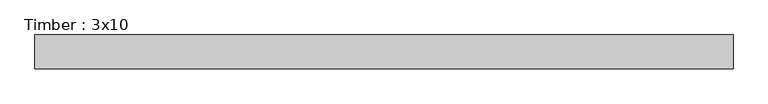
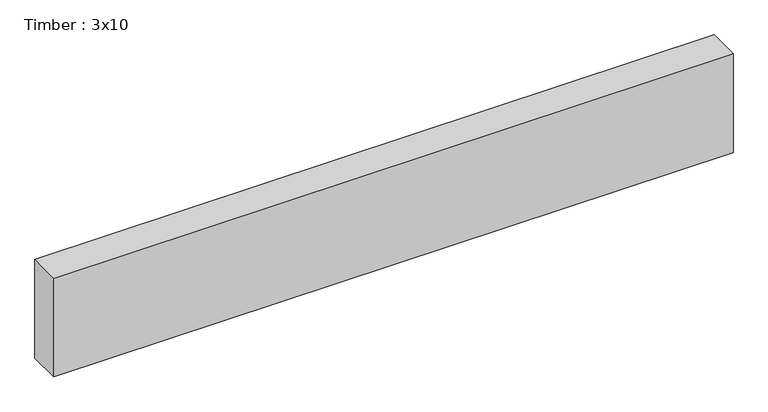
"""IFC4 building model written with IfcOpenShell, lengths in millimetres: beam geometry, Timber : 3x10."""

from ifc_helpers import new_model, si_unit, frame, origin, place, context, project, spatial, polyline, outline, extrude, source, transform, mapped, element, save


def timber_3x10_88a0bdfd(model_context):
    return source(origin(), model_context, "Body", "SweptSolid", [
        extrude(outline(polyline([(785.1325751, 38.1), (785.1325751, -38.1), (-785.1325751, -38.1), (-785.1325751, 38.1), (785.1325751, 38.1)])), frame((0.0, 0.0, -120.65), z_axis=(0.0, 0.0, 1.0), x_axis=(1.0, 0.0, 0.0)), (0.0, 0.0, 1.0), 241.3),
    ])


if __name__ == "__main__":
    model = new_model("IFC4")
    model_context = context("Model", 3, world=origin())
    ifc_project = project(units=[si_unit("LENGTHUNIT", "METRE", prefix="MILLI")], contexts=[model_context])
    site = spatial("IfcSite", under=ifc_project)
    building = spatial("IfcBuilding", under=site)
    placement = place(None, origin())
    timber_3x10_shape = timber_3x10_88a0bdfd(model_context)
    element("IfcBeam", 1, ObjectType="Timber : 3x10", at=placement, inside=building, context=model_context, shape_type="MappedRepresentation", body=[
        mapped(timber_3x10_shape, transform((0.0, 0.0, 0.0), x_axis=(1.0, 0.0, 0.0), y_axis=(0.0, 1.0, 0.0), z_axis=(0.0, 0.0, 1.0))),
    ])
    save(model, "model.ifc")

# Revit data of these elements
# Type "Timber : 3x10"
#   Assembly Code = "B10"
#   A = 0.362847 SF
#   Length [instance default] = 5' - 0"
#   b = 0' - 3"
#   d = 0' - 9 1/2"
#   Structural Material [instance default] = Softwood, Lumber
# Element 1 (IfcBeam, "Timber : 3x10")
#   Materials on its faces: "Softwood, Lumber"
# Materials
#   "Softwood, Lumber": class "Wood", colour RGB 144 113 62, transparency 0, Description = "Pinus Echinata", Cost = 0
